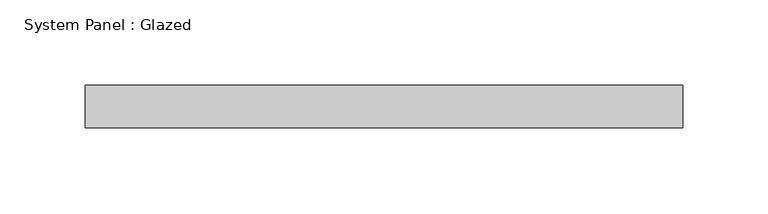
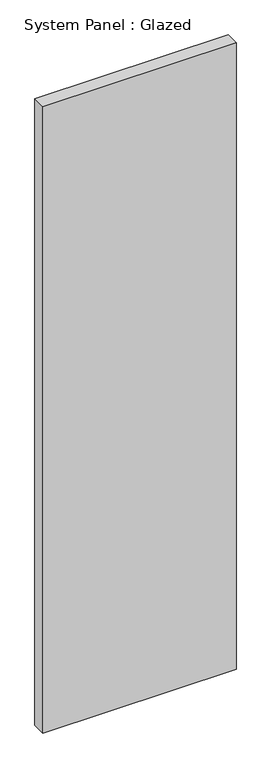
"""IFC4 building model written with IfcOpenShell, lengths in millimetres: plate geometry, System Panel : Glazed."""

from ifc_helpers import new_model, si_unit, origin, origin_with_axes, place, context, project, spatial, polyline, outline, extrude, source, transform, mapped, element, save


def system_panel_glazed_b0a6d7cd(model_context):
    return source(origin(), model_context, "Body", "SweptSolid", [
        extrude(outline(polyline([(175.0, 24.5), (-175.0, 24.5), (-175.0, 49.5), (175.0, 49.5), (175.0, 24.5)])), origin_with_axes(), (0.0, 0.0, 1.0), 1200.0),
    ])


if __name__ == "__main__":
    model = new_model("IFC4")
    model_context = context("Model", 3, world=origin())
    ifc_project = project(units=[si_unit("LENGTHUNIT", "METRE", prefix="MILLI")], contexts=[model_context])
    site = spatial("IfcSite", under=ifc_project)
    building = spatial("IfcBuilding", under=site)
    placement = place(None, origin())
    system_panel_glazed_shape = system_panel_glazed_b0a6d7cd(model_context)
    element("IfcPlate", 1, ObjectType="System Panel : Glazed", at=placement, inside=building, context=model_context, shape_type="MappedRepresentation", body=[
        mapped(system_panel_glazed_shape, transform((0.0, 0.0, 0.0), x_axis=(1.0, 0.0, 0.0), y_axis=(0.0, 1.0, 0.0), z_axis=(0.0, 0.0, 1.0))),
    ])
    save(model, "model.ifc")

# Revit data of these elements
# Element 1 (IfcPlate, "System Panel : Glazed")
#   Materials on its faces: "Glass"
# Materials
#   "Glass": class "Glass", colour RGB 218 227 224, transparency 0.85, Description = "Soda Lime Glass", Cost = 0
